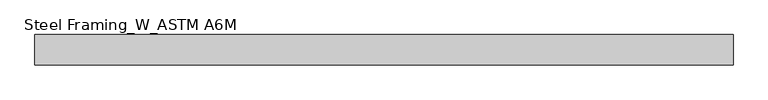
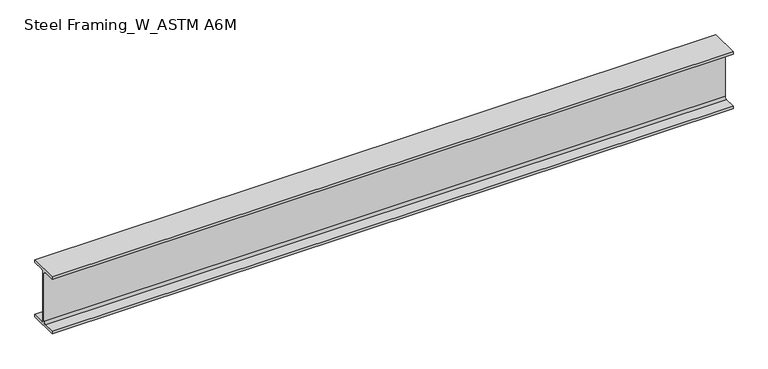
"""IFC4 building model written with IfcOpenShell, lengths in millimetres: beam geometry, Steel Framing_W_ASTM A6M : H_SB_AR_S02_W200x22.5_J1."""

from ifc_helpers import new_model, si_unit, point, frame, frame_2d, origin, place, context, project, spatial, polyline, circle_curve, trimmed, segment, composite_curve, outline, extrude, source, transform, mapped, element, save


def steel_framing_w_astm_a6m_f6c43859(model_context):
    return source(origin(), model_context, "Body", "SweptSolid", [
        extrude(outline(composite_curve([segment(polyline([(51.0, -95.0), (51.0, -103.0), (-51.0, -103.0), (-51.0, -95.0), (-10.71, -95.0)]), True, "CONTINUOUS"), segment(trimmed(circle_curve(frame_2d((-10.71, -87.4)), 7.6), [point((-10.71, -95.0))], [point((-3.11, -87.4))], True, "CARTESIAN"), True, "CONTINUOUS"), segment(polyline([(-3.11, -87.4), (-3.11, 87.4)]), True, "CONTINUOUS"), segment(trimmed(circle_curve(frame_2d((-10.71, 87.4)), 7.6), [point((-3.11, 87.4))], [point((-10.71, 95.0))], True, "CARTESIAN"), True, "CONTINUOUS"), segment(polyline([(-10.71, 95.0), (-51.0, 95.0), (-51.0, 103.0), (51.0, 103.0), (51.0, 95.0), (10.71, 95.0)]), True, "CONTINUOUS"), segment(trimmed(circle_curve(frame_2d((10.71, 87.4)), 7.6), [point((10.71, 95.0))], [point((3.11, 87.4))], True, "CARTESIAN"), True, "CONTINUOUS"), segment(polyline([(3.11, 87.4), (3.11, -87.4)]), True, "CONTINUOUS"), segment(trimmed(circle_curve(frame_2d((10.71, -87.4)), 7.6), [point((3.11, -87.4))], [point((10.71, -95.0))], True, "CARTESIAN"), True, "CONTINUOUS"), segment(polyline([(10.71, -95.0), (51.0, -95.0)]), True, "CONTINUOUS")], self_intersect=False)), frame((-1170.3, 0.0, 0.0), z_axis=(1.0, 0.0, 0.0), x_axis=(0.0, 1.0, 0.0)), (0.0, 0.0, 1.0), 2340.6),
    ])


if __name__ == "__main__":
    model = new_model("IFC4")
    model_context = context("Model", 3, world=origin())
    ifc_project = project(units=[si_unit("LENGTHUNIT", "METRE", prefix="MILLI")], contexts=[model_context])
    site = spatial("IfcSite", under=ifc_project)
    building = spatial("IfcBuilding", under=site)
    placement = place(None, origin())
    steel_framing_w_astm_a6m_shape = steel_framing_w_astm_a6m_f6c43859(model_context)
    element("IfcBeam", 1, ObjectType="Steel Framing_W_ASTM A6M : H_SB_AR_S02_W200x22.5_J1", at=placement, inside=building, context=model_context, shape_type="MappedRepresentation", body=[
        mapped(steel_framing_w_astm_a6m_shape, transform((0.0, 0.0, 0.0), x_axis=(1.0, 0.0, 0.0), y_axis=(0.0, 1.0, 0.0), z_axis=(0.0, 0.0, 1.0))),
    ])
    save(model, "model.ifc")

# Revit data of these elements
# Type "Steel Framing_W_ASTM A6M : H_SB_AR_S02_W200x22.5_J1"
#   Section Name Key = "W8x15"
#   Width = 10.2 cm
#   Web Thickness = 0.622 cm
#   Web Fillet = 0.76 cm
#   Warping Constant = 13900.0 cm⁶
#   Torsional Moment of Inertia = 5.70 cm⁴
#   Section Area = 28.6 cm²
#   Plastic Modulus weak axis = 43.8 cm³
#   Plastic Modulus strong axis = 223.0 cm³
#   Perimeter = 0.795 m²/m
#   Nominal Weight = 22.50 kgf/m
#   Moment of Inertia weak axis = 142.00 cm⁴
#   Moment of Inertia strong axis = 2000.00 cm⁴
#   Height = 20.6 cm
#   Flange Thickness = 0.8 cm
#   Elastic Modulus weak axis = 27.9 cm³
#   Elastic Modulus strong axis = 193.0 cm³
#   Centroid Vertical = 10.3 cm
#   Centroid Horizontal = 5.1 cm
#   Length [instance default] = 1500 mm
#   Structural Material [instance default] = Steel, 45-345
#   Bolt Spacing = 0
#   Assembly Code = ""
# Element 1 (IfcBeam, "Steel Framing_W_ASTM A6M : H_SB_AR_S02_W200x22.5_J1")
#   Materials on its faces: "Steel, 45-345"
# Materials
#   "Steel, 45-345": class "Metal", colour RGB 189 187 185, transparency 0, Description = "Steel 345 MPa", Cost = 0
